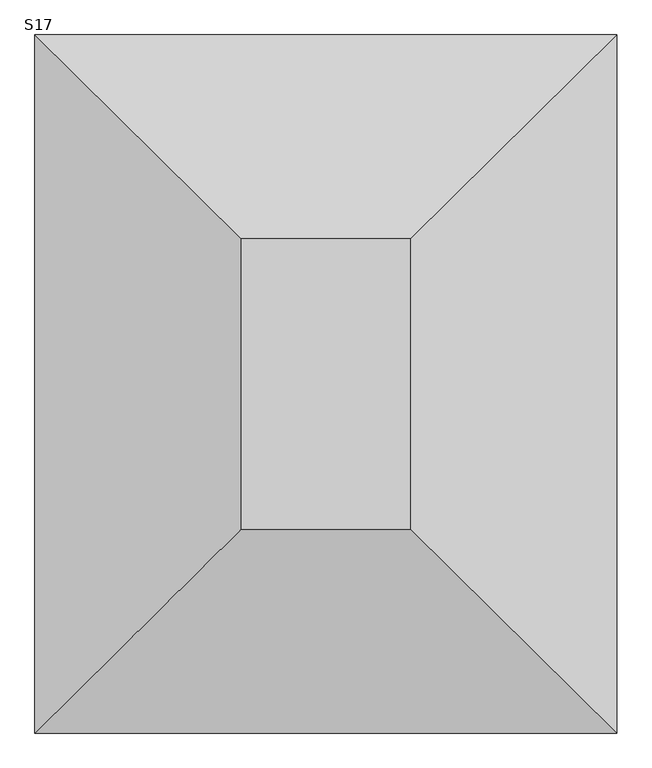
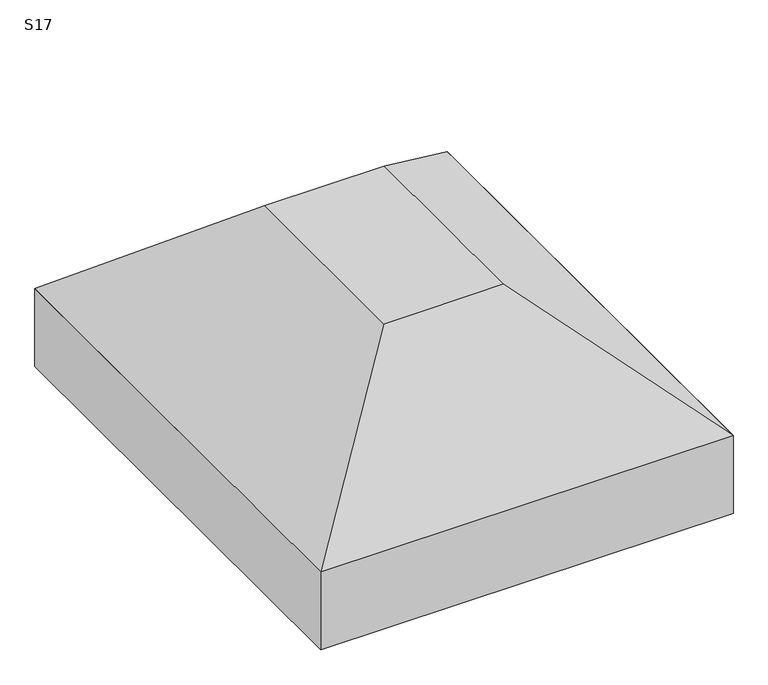
"""IFC4 building model written with IfcOpenShell, lengths in millimetres: fastener geometry, TQS - Sapata : S17."""

from ifc_helpers import new_model, si_unit, frame, origin, place, context, project, spatial, polyline, outline, extrude, faceted_brep, source, transform, mapped, element, save


def s17_fc997501(model_context):
    return source(origin(), model_context, "Body", "SolidModel", [
        faceted_brep([(-55.0, 50.0, 0.0), (-345.0, 50.0, 0.0), (-345.0, -450.0, 0.0), (-55.0, -450.0, 0.0), (300.0, 400.0, -300.0), (300.0, -800.0, -300.0), (-700.0, -800.0, -300.0), (-700.0, 400.0, -300.0)], [[[0, 1, 2, 3]], [[4, 5, 6, 7]], [[4, 7, 1, 0]], [[7, 6, 2, 1]], [[6, 5, 3, 2]], [[5, 4, 0, 3]]]),
        extrude(outline(polyline([(300.0, 400.0), (300.0, -800.0), (-700.0, -800.0), (-700.0, 400.0), (300.0, 400.0)])), frame((0.0, 0.0, -500.0), z_axis=(0.0, 0.0, 1.0), x_axis=(1.0, 0.0, 0.0)), (0.0, 0.0, 1.0), 200.0),
    ])


if __name__ == "__main__":
    model = new_model("IFC4")
    model_context = context("Model", 3, world=origin())
    ifc_project = project(units=[si_unit("LENGTHUNIT", "METRE", prefix="MILLI")], contexts=[model_context])
    site = spatial("IfcSite", under=ifc_project)
    building = spatial("IfcBuilding", under=site)
    placement = place(None, origin())
    s17_shape = s17_fc997501(model_context)
    element("IfcFastener", 1, ObjectType="TQS - Sapata : S17", at=placement, inside=building, context=model_context, shape_type="MappedRepresentation", body=[
        mapped(s17_shape, transform((0.0, 0.0, 0.0), x_axis=(1.0, 0.0, 0.0), y_axis=(0.0, 1.0, 0.0), z_axis=(0.0, 0.0, 1.0))),
    ])
    save(model, "model.ifc")

# Revit data of these elements
# Type "TQS - Sapata : S17"
#   TY = 0.50 m
#   TX = 0.29 m
#   HS = 0.50 m
#   H0 = 0.20 m
#   EXCYABS = 0.60 m
#   EXCY = 0.00 m
#   EXCXABS = 0.50 m
#   EXCX = 0.00 m
#   DIMY = 1.20 m
#   DIMX = 1.00 m
#   Material estrutural = Concreto - Concreto concretado no local
#   Width = 0
#   Length = 0
# Element 1 (IfcFastener, "TQS - Sapata : S17")
#   Materials on its faces: "Concreto - Concreto concretado no local"
# Materials
#   "Concreto - Concreto concretado no local": class "Concreto", colour RGB 192 192 192, transparency 0
